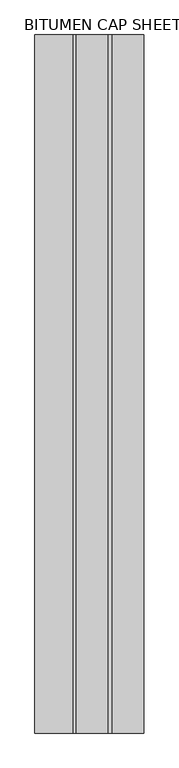
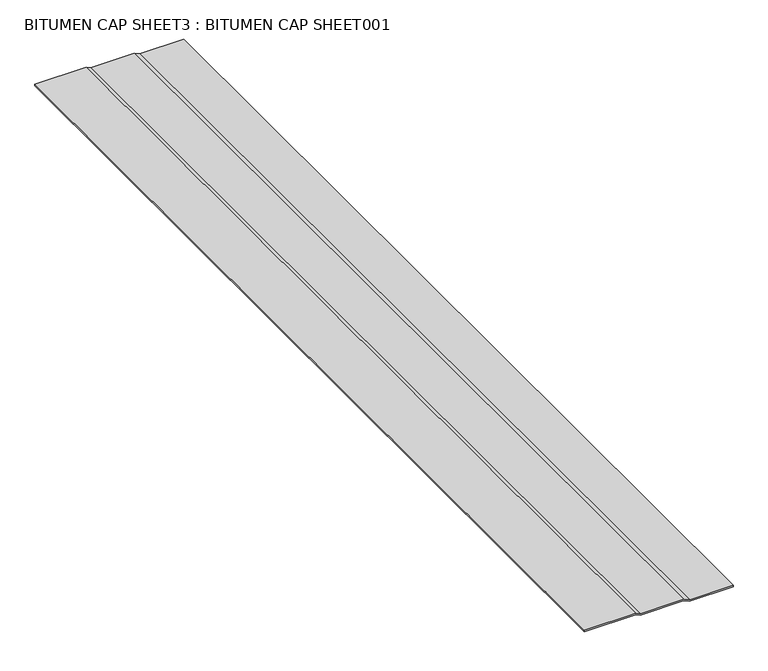
"""IFC4 building model written with IfcOpenShell, lengths in millimetres: proxy geometry, BITUMEN CAP SHEET3 : BITUMEN CAP SHEET001."""

from ifc_helpers import new_model, si_unit, frame, origin, place, context, project, spatial, polyline, outline, extrude, source, transform, mapped, element, save


def bitumen_cap_sheet3_bitumen_cap_sheet001_3f8c56e2(model_context):
    return source(origin(), model_context, "Body", "SweptSolid", [
        extrude(outline(polyline([(40259.2002678, -4699.8063764), (40262.3752678, -4699.8063764), (40262.3752678, -4791.325638), (40267.6612773, -4803.7904566), (40267.6612773, -4894.4742123), (40271.9940719, -4904.1911138), (40271.9940719, -5012.0776104), (40268.8188423, -5012.0776104), (40268.8188423, -4904.8663993), (40264.4862773, -4895.1500128), (40264.4862773, -4804.4358566), (40259.2002678, -4791.971038), (40259.2002678, -4699.8063764)])), frame((0.0, -1052.8906574, 0.0), z_axis=(0.0, 1.0, 0.0), x_axis=(0.0, 0.0, 1.0)), (0.0, 0.0, 1.0), 2000.25),
    ])


if __name__ == "__main__":
    model = new_model("IFC4")
    model_context = context("Model", 3, world=origin())
    ifc_project = project(units=[si_unit("LENGTHUNIT", "METRE", prefix="MILLI")], contexts=[model_context])
    site = spatial("IfcSite", under=ifc_project)
    building = spatial("IfcBuilding", under=site)
    placement = place(None, origin())
    bitumen_cap_sheet3_bitumen_cap_sheet001_shape = bitumen_cap_sheet3_bitumen_cap_sheet001_3f8c56e2(model_context)
    element("IfcBuildingElementProxy", 1, Name="BITUMEN CAP SHEET3 : BITUMEN CAP SHEET001", ObjectType="BITUMEN CAP SHEET3 : BITUMEN CAP SHEET001", at=placement, inside=building, context=model_context, shape_type="MappedRepresentation", body=[
        mapped(bitumen_cap_sheet3_bitumen_cap_sheet001_shape, transform((0.0, 0.0, 0.0), x_axis=(1.0, 0.0, 0.0), y_axis=(0.0, 1.0, 0.0), z_axis=(0.0, 0.0, 1.0))),
    ])
    save(model, "model.ifc")

# Revit data of these elements
# Type "BITUMEN CAP SHEET3 : BITUMEN CAP SHEET001"
#   NameOverride = "BITUMEN CAP SHEET001"
# Element 1 (IfcBuildingElementProxy, "BITUMEN CAP SHEET3 : BITUMEN CAP SHEET001")
#   Materials on its faces: "MODIFIED BITUMEN GRANULE SURFACED CAP SHEET"
# Materials
#   "MODIFIED BITUMEN GRANULE SURFACED CAP SHEET": class "Unassigned", colour RGB 85 85 127, transparency 0
